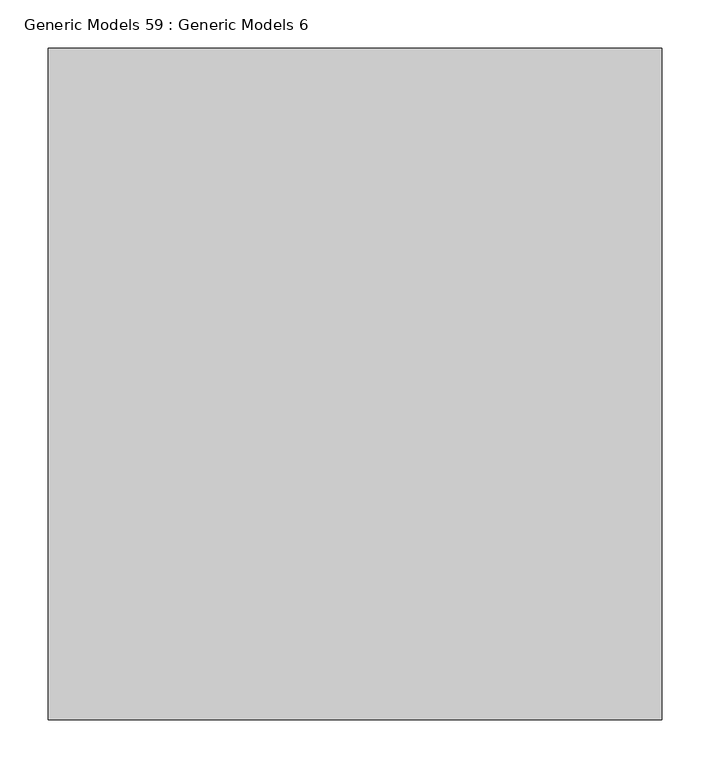
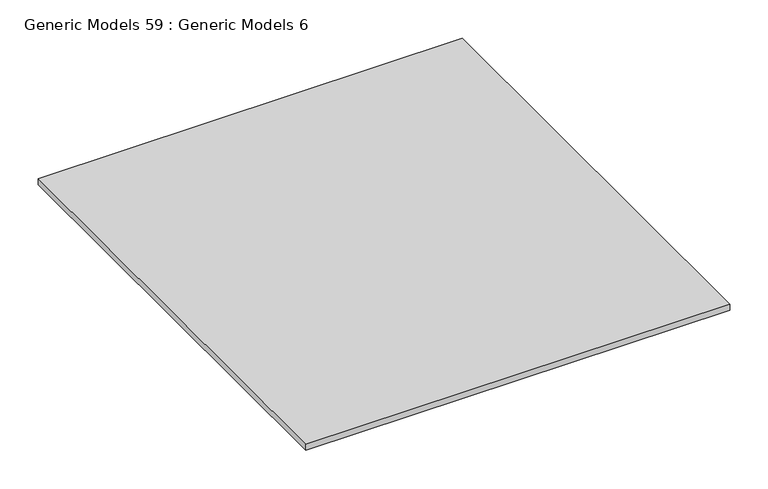
"""IFC4 building model written with IfcOpenShell, lengths in millimetres: proxy geometry, Generic Models 59 : Generic Models 6."""

from ifc_helpers import new_model, si_unit, frame, origin, place, context, project, spatial, polyline, outline, extrude, source, transform, mapped, element, save


def generic_models_59_generic_models_6_5b47f486(model_context):
    return source(origin(), model_context, "Body", "SweptSolid", [
        extrude(outline(polyline([(1257.1263704, 1781.5884092), (1893.509978, 1781.5884092), (1893.509978, 1085.5309662), (1257.1263704, 1085.5309662), (1257.1263704, 1781.5884092)])), frame((0.0, 0.0, 123450.096), z_axis=(0.0, 0.0, 1.0), x_axis=(1.0, 0.0, 0.0)), (0.0, 0.0, 1.0), 9.525),
    ])


if __name__ == "__main__":
    model = new_model("IFC4")
    model_context = context("Model", 3, world=origin())
    ifc_project = project(units=[si_unit("LENGTHUNIT", "METRE", prefix="MILLI")], contexts=[model_context])
    site = spatial("IfcSite", under=ifc_project)
    building = spatial("IfcBuilding", under=site)
    placement = place(None, origin())
    generic_models_59_generic_models_6_shape = generic_models_59_generic_models_6_5b47f486(model_context)
    element("IfcBuildingElementProxy", 1, Name="Generic Models 59 : Generic Models 6", ObjectType="Generic Models 59 : Generic Models 6", at=placement, inside=building, context=model_context, shape_type="MappedRepresentation", body=[
        mapped(generic_models_59_generic_models_6_shape, transform((0.0, 0.0, 0.0), x_axis=(1.0, 0.0, 0.0), y_axis=(0.0, 1.0, 0.0), z_axis=(0.0, 0.0, 1.0))),
    ])
    save(model, "model.ifc")

# Revit data of these elements
# Element 1 (IfcBuildingElementProxy, "Generic Models 59 : Generic Models 6")
#   Materials on its faces: "_MORTAR SETTING BED"
# Materials
#   "_MORTAR SETTING BED": class "Generic", colour RGB 191 191 191, transparency 0, Cost = 0
